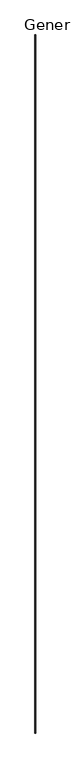
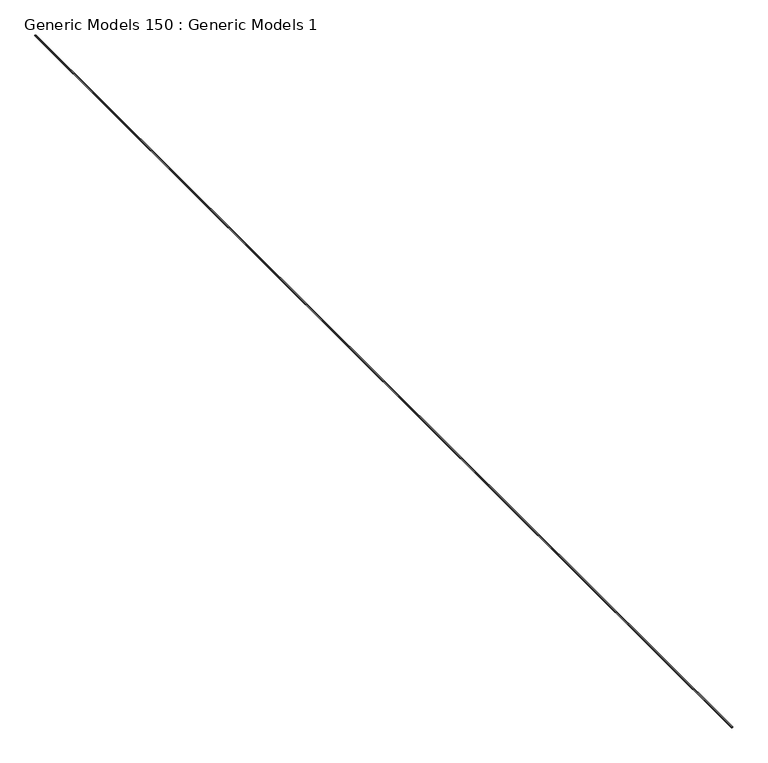
"""IFC4 building model written with IfcOpenShell, lengths in millimetres: proxy geometry, Generic Models 150 : Generic Models 1."""

from ifc_helpers import new_model, si_unit, point, frame, origin, place, context, project, spatial, polyline, circle_curve, ellipse_curve, trimmed, source, transform, mapped, element, save
from ifc_brep_helpers import plane_surface, cylinder_surface, revolved_surface, extruded_surface, advanced_brep


def generic_models_150_generic_models_1_cef9da7c(model_context):
    return source(origin(), model_context, "Body", "AdvancedBrep", [
        advanced_brep(
        [(-6651.2562339, 11981.8769662, 126151.8372608), (-6651.2562339, 11981.8769662, 126161.3622608), (-6646.4937339, 11981.8769662, 126161.3622608), (-6645.0660949, 11981.8769662, 126159.456273), (-6645.0660949, 11981.8769662, 126153.7432487), (-6646.4937339, 11981.8769662, 126151.8372608), (-6651.2562339, -7068.1230338, 126151.8372608), (-6646.4937339, -7068.1230338, 126151.8372608), (-6645.0660949, -7068.1230338, 126153.7432487), (-6645.0660949, -7068.1230338, 126159.456273), (-6646.4937339, -7068.1230338, 126161.3622608), (-6651.2562339, -7068.1230338, 126161.3622608)],
        [
            (0, 1, circle_curve(frame((-6655.6283446, 11981.8769662, 126156.5997608), z_axis=(0.0, -1.0, 0.0), x_axis=(0.0, 0.0, -1.0)), 6.4650413)),
            (1, 2),
            (2, 3, circle_curve(frame((-6650.8658446, 11981.8769662, 126156.5997608), z_axis=(0.0, 1.0, 0.0), x_axis=(0.0, 0.0, -1.0)), 6.4650413)),
            (3, 4, ellipse_curve(frame((-6639.3499839, 11981.8769662, 126156.5997608), z_axis=(0.0, 1.0, 0.0), x_axis=(-1.0, 0.0, 0.0)), 7.14375, 4.7625)),
            (4, 5, circle_curve(frame((-6650.8658446, 11981.8769662, 126156.5997608), z_axis=(0.0, 1.0, 0.0), x_axis=(0.0, 0.0, -1.0)), 6.4650413)),
            (5, 0),
            (6, 7),
            (7, 8, circle_curve(frame((-6650.8658446, -7068.1230338, 126156.5997608), z_axis=(0.0, -1.0, 0.0), x_axis=(0.0, 0.0, -1.0)), 6.4650413)),
            (8, 9, ellipse_curve(frame((-6639.3499839, -7068.1230338, 126156.5997608), z_axis=(0.0, -1.0, 0.0), x_axis=(-1.0, 0.0, 0.0)), 7.14375, 4.7625)),
            (9, 10, circle_curve(frame((-6650.8658446, -7068.1230338, 126156.5997608), z_axis=(0.0, -1.0, 0.0), x_axis=(0.0, 0.0, -1.0)), 6.4650413)),
            (10, 11),
            (11, 6, circle_curve(frame((-6655.6283446, -7068.1230338, 126156.5997608), z_axis=(0.0, 1.0, 0.0), x_axis=(0.0, 0.0, -1.0)), 6.4650413)),
            (3, 9),
            (8, 4),
            (0, 6),
            (11, 1),
            (10, 2),
            (7, 5),
        ],
        [
            plane_surface(frame((-6651.2562339, 11981.8769662, 126161.3622608), z_axis=(0.0, 1.0, 0.0), x_axis=(-1.0, 0.0, 0.0))),
            plane_surface(frame((-6651.2562339, -7068.1230338, 126161.3622608), z_axis=(0.0, -1.0, 0.0), x_axis=(-1.0, 0.0, 0.0))),
            extruded_surface(trimmed(ellipse_curve(frame((-6639.3499839, -7068.1230338, 126156.5997608), z_axis=(0.0, 1.0, 0.0), x_axis=(-1.0, 0.0, 0.0)), 7.14375, 4.7625), [point((-6645.0660949, -7068.1230338, 126159.456273))], [point((-6645.0660949, -7068.1230338, 126153.7432487))], True, "CARTESIAN"), (0.0, 19050.0, 0.0), 19050.0),
            revolved_surface(polyline([(-6655.6283446, -7068.1230338000005, 126150.1347195), (-6655.6283446, 11981.8769662, 126150.1347195)]), (-6655.6283446, 11981.8769662, 126156.5997608), (0.0, -1.0, 0.0)),
            plane_surface(frame((-6651.2562339, 11981.8769662, 126161.3622608), z_axis=(0.0, 0.0, 1.0), x_axis=(0.0, -1.0, 0.0))),
            cylinder_surface(frame((-6650.8658446, 11981.8769662, 126156.5997608), z_axis=(0.0, 1.0, 0.0), x_axis=(0.0, 0.0, -1.0)), 6.4650413),
            plane_surface(frame((-6646.4937339, 11981.8769662, 126151.8372608), z_axis=(0.0, 0.0, -1.0), x_axis=(0.0, -1.0, 0.0))),
        ],
        [
            (0, [[1, 2, 3, 4, 5, 6]]),
            (1, [[7, 8, 9, 10, 11, 12]]),
            (2, [[-4, 13, -9, 14]]),
            (3, [[-1, 15, -12, 16]]),
            (4, [[-2, -16, -11, 17]]),
            (5, [[-3, -17, -10, -13]]),
            (5, [[-5, -14, -8, 18]]),
            (6, [[-6, -18, -7, -15]]),
        ],
    ),
    ])


if __name__ == "__main__":
    model = new_model("IFC4")
    model_context = context("Model", 3, world=origin())
    ifc_project = project(units=[si_unit("LENGTHUNIT", "METRE", prefix="MILLI")], contexts=[model_context])
    site = spatial("IfcSite", under=ifc_project)
    building = spatial("IfcBuilding", under=site)
    placement = place(None, origin())
    generic_models_150_generic_models_1_shape = generic_models_150_generic_models_1_cef9da7c(model_context)
    element("IfcBuildingElementProxy", 1, Name="Generic Models 150 : Generic Models 1", ObjectType="Generic Models 150 : Generic Models 1", at=placement, inside=building, context=model_context, shape_type="MappedRepresentation", body=[
        mapped(generic_models_150_generic_models_1_shape, transform((0.0, 0.0, 0.0), x_axis=(1.0, 0.0, 0.0), y_axis=(0.0, 1.0, 0.0), z_axis=(0.0, 0.0, 1.0))),
    ])
    save(model, "model.ifc")

# Revit data of these elements
# Element 1 (IfcBuildingElementProxy, "Generic Models 150 : Generic Models 1")
#   Materials on its faces: "_SEALANT AND BACKROD, IF NECESSARY"
# Materials
#   "_SEALANT AND BACKROD, IF NECESSARY": class "Generic", colour RGB 190 220 196, transparency 0, Cost = 0
